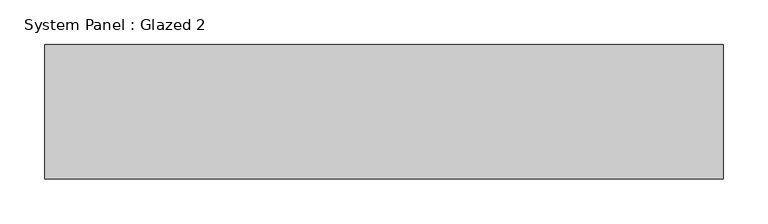
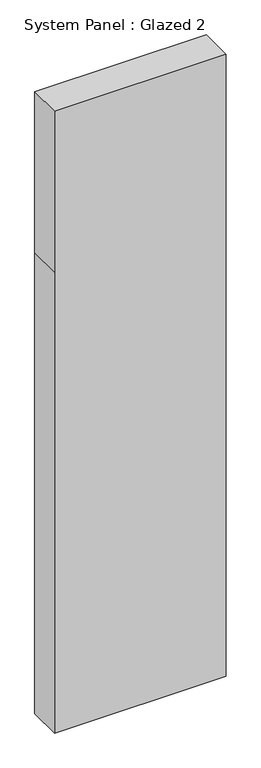
"""IFC4 building model written with IfcOpenShell, lengths in millimetres: plate geometry, System Panel : Glazed 2."""

from ifc_helpers import new_model, si_unit, frame, origin, place, context, project, spatial, polyline, outline, extrude, source, transform, mapped, element, save


def system_panel_glazed_2_4537a6f7(model_context):
    return source(origin(), model_context, "Body", "SweptSolid", [
        extrude(outline(polyline([(0.0, -379.0), (0.0, 379.0), (2150.0, 379.0), (2900.0, 379.0), (2900.0, -379.0), (2150.0, -379.0), (0.0, -379.0)])), frame((0.0, -75.0, 0.0), z_axis=(0.0, 1.0, 0.0), x_axis=(0.0, 0.0, 1.0)), (0.0, 0.0, 1.0), 150.0),
    ])


if __name__ == "__main__":
    model = new_model("IFC4")
    model_context = context("Model", 3, world=origin())
    ifc_project = project(units=[si_unit("LENGTHUNIT", "METRE", prefix="MILLI")], contexts=[model_context])
    site = spatial("IfcSite", under=ifc_project)
    building = spatial("IfcBuilding", under=site)
    placement = place(None, origin())
    system_panel_glazed_2_shape = system_panel_glazed_2_4537a6f7(model_context)
    element("IfcPlate", 1, ObjectType="System Panel : Glazed 2", at=placement, inside=building, context=model_context, shape_type="MappedRepresentation", body=[
        mapped(system_panel_glazed_2_shape, transform((0.0, 0.0, 0.0), x_axis=(1.0, 0.0, 0.0), y_axis=(0.0, 1.0, 0.0), z_axis=(0.0, 0.0, 1.0))),
    ])
    save(model, "model.ifc")

# Revit data of these elements
# Type "System Panel : Glazed 2"
#   COBie.Type = no
# Element 1 (IfcPlate, "System Panel : Glazed 2")
#   Materials on its faces: "Glass"
# Materials
#   "Glass": class "Glass", colour RGB 0 128 192, transparency 0.75, Description = "Soda Lime Glass", Cost = 0
